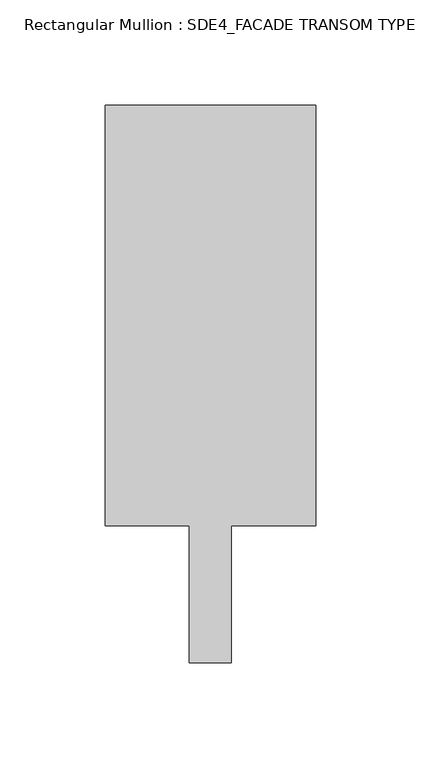
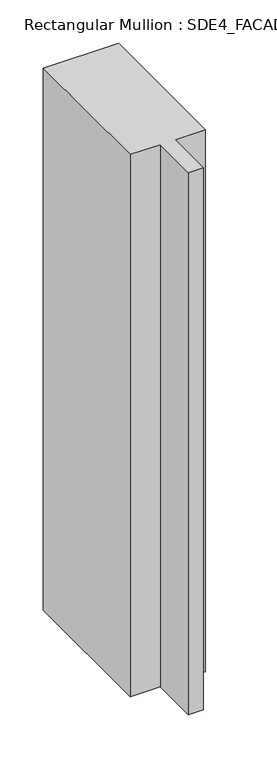
"""IFC4 building model written with IfcOpenShell, lengths in millimetres: member geometry, Rectangular Mullion : SDE4_FACADE TRANSOM TYPE 2."""

from ifc_helpers import new_model, si_unit, frame, origin, place, context, project, spatial, polyline, outline, extrude, source, transform, mapped, element, save


def rectangular_mullion_sde4_facade_transom_type_2_7a017769(model_context):
    return source(origin(), model_context, "Body", "SweptSolid", [
        extrude(outline(polyline([(50.0, 132.5), (50.0, -67.5), (10.0, -67.5), (10.0, -132.5), (-10.0, -132.5), (-10.0, -67.5), (-50.0, -67.5), (-50.0, 132.5), (50.0, 132.5)])), frame((0.0, 0.0, -762.8193467), z_axis=(0.0, 0.0, 1.0), x_axis=(1.0, 0.0, 0.0)), (0.0, 0.0, 1.0), 762.8193467),
    ])


if __name__ == "__main__":
    model = new_model("IFC4")
    model_context = context("Model", 3, world=origin())
    ifc_project = project(units=[si_unit("LENGTHUNIT", "METRE", prefix="MILLI")], contexts=[model_context])
    site = spatial("IfcSite", under=ifc_project)
    building = spatial("IfcBuilding", under=site)
    placement = place(None, origin())
    rectangular_mullion_sde4_facade_transom_type_2_shape = rectangular_mullion_sde4_facade_transom_type_2_7a017769(model_context)
    element("IfcMember", 1, ObjectType="Rectangular Mullion : SDE4_FACADE TRANSOM TYPE 2", at=placement, inside=building, context=model_context, shape_type="MappedRepresentation", body=[
        mapped(rectangular_mullion_sde4_facade_transom_type_2_shape, transform((0.0, 0.0, 0.0), x_axis=(1.0, 0.0, 0.0), y_axis=(0.0, 1.0, 0.0), z_axis=(0.0, 0.0, 1.0))),
    ])
    save(model, "model.ifc")

# Revit data of these elements
# Type "Rectangular Mullion : SDE4_FACADE TRANSOM TYPE 2"
#   built-in parameter 1007322 = 0.869423 (stored number, unit not read)
#   built-in parameter 1007321 = 0.164042 (stored number, unit not read)
#   built-in parameter 1007320 = 0.164042 (stored number, unit not read)
